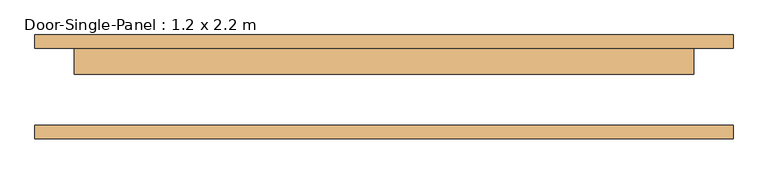
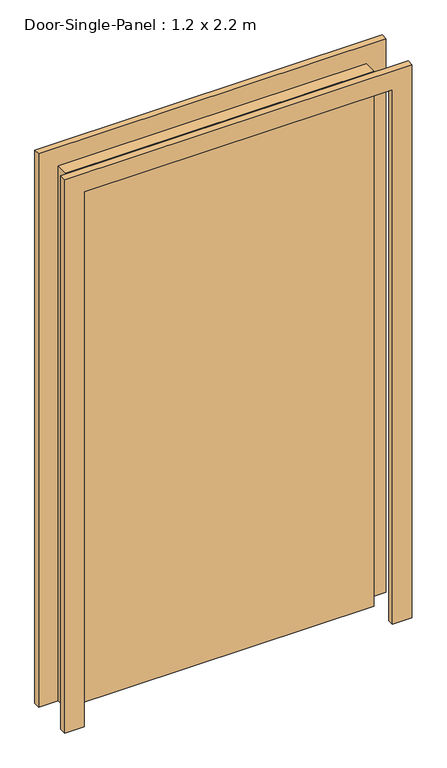
"""IFC4 building model written with IfcOpenShell, lengths in millimetres: door geometry, Door-Single-Panel : 1.2 x 2.2 m."""

import ifcopenshell
import ifcopenshell.guid

model = None  # the IFC model being written
_history = None  # IfcOwnerHistory: only IFC2X3 demands one
_inside = {}  # id of a spatial element -> (the spatial element, [elements in it])
_under = {}  # id of a project, library or spatial element -> (it, [spatial elements below it])
_declared = {}  # id of a project -> (the project, [libraries it declares])
_typed = {}  # id of a type object -> (the type object, [elements of that type])
_made_of = {}  # id of a material, layer set ... -> (it, [elements and type objects made of it])


def new_model(schema):
    """Start an empty IFC model of exactly this schema.

    Asked for "IFC4X3", IfcOpenShell would pick the latest addendum, in which some entities
    have other attributes; the version numbers below select the first issue.
    IFC2X3 requires an IfcOwnerHistory on every rooted entity: one is made here for all.
    """
    global model, _history
    if schema == "IFC4X3":
        model = ifcopenshell.file(schema_version=(4, 3, 0, 0))
    else:
        model = ifcopenshell.file(schema=schema)
    _inside.clear()
    _under.clear()
    _declared.clear()
    _typed.clear()
    _made_of.clear()
    _history = None
    if model.schema == "IFC2X3":
        org = make("IfcOrganization", Name="unknown")
        user = make(
            "IfcPersonAndOrganization",
            ThePerson=make("IfcPerson", FamilyName="unknown"),
            TheOrganization=org,
        )
        app = make(
            "IfcApplication",
            ApplicationDeveloper=org,
            Version="unknown",
            ApplicationFullName="unknown",
            ApplicationIdentifier="unknown",
        )
        _history = make(
            "IfcOwnerHistory",
            OwningUser=user,
            OwningApplication=app,
            ChangeAction="ADDED",
            CreationDate=0,
        )
    return model


def make(cls, **values):
    """One entity of the class cls with the attributes given. An attribute that is None is left unset."""
    return model.create_entity(
        cls, **{name: value for name, value in values.items() if value is not None}
    )


def rooted(cls, **values):
    """An entity with a GlobalId (a new one), such as an element, a storey or a relation."""
    return make(cls, GlobalId=ifcopenshell.guid.new(), OwnerHistory=_history, **values)


def si_unit(unit_type, name, prefix=None):
    """IfcSIUnit, for example si_unit("LENGTHUNIT", "METRE", prefix="MILLI")."""
    return make("IfcSIUnit", UnitType=unit_type, Prefix=prefix, Name=name)


def assignment(units):
    """IfcUnitAssignment: the units of a project."""
    return None if units is None else make("IfcUnitAssignment", Units=units)


def point(xyz):
    """IfcCartesianPoint."""
    return None if xyz is None else make("IfcCartesianPoint", Coordinates=xyz)


def direction(xyz):
    """IfcDirection."""
    return None if xyz is None else make("IfcDirection", DirectionRatios=xyz)


def frame(location, z_axis=None, x_axis=None):
    """IfcAxis2Placement3D, a coordinate frame: its origin and axes. An axis left out is left unset."""
    return make(
        "IfcAxis2Placement3D",
        Location=point(location),
        Axis=direction(z_axis),
        RefDirection=direction(x_axis),
    )


def origin():
    """The frame at (0, 0, 0) with its axes left unset."""
    return frame((0.0, 0.0, 0.0))


def origin_with_axes():
    """The frame at (0, 0, 0) with the z axis (0, 0, 1) and the x axis (1, 0, 0) written out."""
    return frame((0.0, 0.0, 0.0), z_axis=(0.0, 0.0, 1.0), x_axis=(1.0, 0.0, 0.0))


def place(relative_to, where):
    """IfcLocalPlacement: puts the frame where relative to a parent placement (None: the world)."""
    return make(
        "IfcLocalPlacement", PlacementRelTo=relative_to, RelativePlacement=where
    )


def context(
    kind, dimensions, precision=None, world=None, true_north=None, identifier=None
):
    """IfcGeometricRepresentationContext, for example the 3D "Model" context."""
    return make(
        "IfcGeometricRepresentationContext",
        ContextIdentifier=identifier,
        ContextType=kind,
        CoordinateSpaceDimension=dimensions,
        Precision=precision,
        WorldCoordinateSystem=world,
        TrueNorth=true_north,
    )


def project(units=None, contexts=None):
    """IfcProject with its units and contexts."""
    return rooted(
        "IfcProject",
        Name="project",
        RepresentationContexts=contexts,
        UnitsInContext=assignment(units),
    )


def spatial(cls, under=None, at=None, **own):
    """A site, building, storey or space (cls), placed at a placement, below another one or the project."""
    s = rooted(cls, ObjectPlacement=at, **own)
    if under is not None:
        _under.setdefault(under.id(), (under, []))[1].append(s)
    return s


def polyline(points):
    """IfcPolyline through the points."""
    return make("IfcPolyline", Points=[point(p) for p in points])


def outline(outer, holes=None, kind="AREA"):
    """IfcArbitraryClosedProfileDef: a profile drawn as a closed curve; with holes, ...WithVoids."""
    if holes is None:
        return make("IfcArbitraryClosedProfileDef", ProfileType=kind, OuterCurve=outer)
    return make(
        "IfcArbitraryProfileDefWithVoids",
        ProfileType=kind,
        OuterCurve=outer,
        InnerCurves=holes,
    )


def extrude(swept, where, along, depth):
    """IfcExtrudedAreaSolid: the profile swept, set in the frame where, extruded along a direction by depth."""
    return make(
        "IfcExtrudedAreaSolid",
        SweptArea=swept,
        Position=where,
        ExtrudedDirection=direction(along),
        Depth=depth,
    )


def shape(context_of_items, identifier, shape_type, items):
    """IfcShapeRepresentation: the items that make up one representation, for example the "Body"."""
    return make(
        "IfcShapeRepresentation",
        ContextOfItems=context_of_items,
        RepresentationIdentifier=identifier,
        RepresentationType=shape_type,
        Items=items,
    )


def source(mapping_origin, context_of_items, identifier, shape_type, items):
    """IfcRepresentationMap: a shape defined once, which mapped items show again and again."""
    return make(
        "IfcRepresentationMap",
        MappingOrigin=mapping_origin,
        MappedRepresentation=shape(context_of_items, identifier, shape_type, items),
    )


def transform(
    local_origin,
    x_axis=None,
    y_axis=None,
    z_axis=None,
    scale=None,
    scale2=None,
    scale3=None,
    uniform=True,
):
    """IfcCartesianTransformationOperator3D, or its non-uniform kind. x_axis, y_axis, z_axis: its Axis1, 2, 3."""
    if uniform:
        return make(
            "IfcCartesianTransformationOperator3D",
            Axis1=direction(x_axis),
            Axis2=direction(y_axis),
            LocalOrigin=point(local_origin),
            Scale=scale,
            Axis3=direction(z_axis),
        )
    return make(
        "IfcCartesianTransformationOperator3DnonUniform",
        Axis1=direction(x_axis),
        Axis2=direction(y_axis),
        LocalOrigin=point(local_origin),
        Scale=scale,
        Axis3=direction(z_axis),
        Scale2=scale2,
        Scale3=scale3,
    )


def mapped(mapping_source, mapping_target):
    """IfcMappedItem: shows the shape of a source again, moved by a transform."""
    return make(
        "IfcMappedItem", MappingSource=mapping_source, MappingTarget=mapping_target
    )


def made_of(thing, what):
    """Note that an element or type object is made of a material, layer set ...; save() writes the relation."""
    if what is not None:
        _made_of.setdefault(what.id(), (what, []))[1].append(thing)
    return thing


def element(
    cls,
    number,
    at=None,
    inside=None,
    cuts=None,
    type_object=None,
    material=None,
    context=None,
    identifier="Body",
    shape_type=None,
    held_by="IfcProductDefinitionShape",
    body=None,
    shapes=None,
    **own,
):
    """One element of the class cls, such as IfcWall. Its Tag is "e" and its number.

    at: its placement. inside: the storey or other place that contains it. cuts: it is an
    opening in that element (IfcRelVoidsElement). A single representation is given by context,
    identifier, shape_type and body (its items); several are given by shapes. held_by: the class
    of the entity that holds the representations. save() writes the other relations.
    """
    e = rooted(cls, Tag="e%d" % number, ObjectPlacement=at, **own)
    if body is not None:
        shapes = [shape(context, identifier, shape_type, body)]
    if shapes is not None:
        e.Representation = make(held_by, Representations=shapes)
    if inside is not None:
        _inside.setdefault(inside.id(), (inside, []))[1].append(e)
    if cuts is not None:
        rooted(
            "IfcRelVoidsElement", RelatingBuildingElement=cuts, RelatedOpeningElement=e
        )
    if type_object is not None:
        _typed.setdefault(type_object.id(), (type_object, []))[1].append(e)
    return made_of(e, material)


def aggregate(whole, parts):
    """IfcRelAggregates: a whole, such as a stair, and the parts it consists of."""
    return rooted("IfcRelAggregates", RelatingObject=whole, RelatedObjects=parts)


def save(model, path):
    """Write the relations noted so far, then the file.

    IfcRelAggregates (storeys below a building ...), IfcRelContainedInSpatialStructure (elements
    in a storey), IfcRelDefinesByType, IfcRelAssociatesMaterial and IfcRelDeclares: one each for
    every whole, place, type object, material and project.
    """
    for whole, parts in _under.values():
        aggregate(whole, parts)
    for where, things in _inside.values():
        rooted(
            "IfcRelContainedInSpatialStructure",
            RelatedElements=things,
            RelatingStructure=where,
        )
    for kind, things in _typed.values():
        rooted("IfcRelDefinesByType", RelatedObjects=things, RelatingType=kind)
    for what, things in _made_of.values():
        rooted("IfcRelAssociatesMaterial", RelatedObjects=things, RelatingMaterial=what)
    for by, libraries in _declared.values():
        rooted("IfcRelDeclares", RelatingContext=by, RelatedDefinitions=libraries)
    model.write(path)


def door_single_panel_1_2_x_2_2_m_37493633(model_context):
    return source(origin(), model_context, "Body", "SweptSolid", [
        extrude(outline(polyline([(600.0, 24.2), (-600.0, 24.2), (-600.0, 75.0), (600.0, 75.0), (600.0, 24.2)])), origin_with_axes(), (0.0, 0.0, 1.0), 2200.0),
        extrude(outline(polyline([(2276.2, 676.2), (2276.2, -676.2), (0.0, -676.2), (0.0, -600.0), (2200.0, -600.0), (2200.0, 600.0), (0.0, 600.0), (0.0, 676.2), (2276.2, 676.2)])), frame((0.0, -100.4, 0.0), z_axis=(0.0, 1.0, 0.0), x_axis=(0.0, 0.0, 1.0)), (0.0, 0.0, 1.0), 25.4),
        extrude(outline(polyline([(2276.2, -676.2), (0.0, -676.2), (0.0, -600.0), (2200.0, -600.0), (2200.0, 600.0), (0.0, 600.0), (0.0, 676.2), (2276.2, 676.2), (2276.2, -676.2)])), frame((0.0, 75.0, 0.0), z_axis=(0.0, 1.0, 0.0), x_axis=(0.0, 0.0, 1.0)), (0.0, 0.0, 1.0), 25.4),
    ])


if __name__ == "__main__":
    model = new_model("IFC4")
    model_context = context("Model", 3, world=origin())
    ifc_project = project(units=[si_unit("LENGTHUNIT", "METRE", prefix="MILLI")], contexts=[model_context])
    site = spatial("IfcSite", under=ifc_project)
    building = spatial("IfcBuilding", under=site)
    placement = place(None, origin())
    door_single_panel_1_2_x_2_2_m_shape = door_single_panel_1_2_x_2_2_m_37493633(model_context)
    element("IfcDoor", 1, ObjectType="Door-Single-Panel : 1.2 x 2.2 m", at=placement, inside=building, context=model_context, shape_type="MappedRepresentation", body=[
        mapped(door_single_panel_1_2_x_2_2_m_shape, transform((0.0, 0.0, 0.0), x_axis=(1.0, 0.0, 0.0), y_axis=(0.0, 1.0, 0.0), z_axis=(0.0, 0.0, 1.0))),
    ])
    save(model, "model.ifc")

# Revit data of these elements
# Type "Door-Single-Panel : 1.2 x 2.2 m"
#   Type Mark = "47"
#   Construction Type Id = "DOOR"
#   Analytic Construction = "Wooden"
#   Thickness = 0.0508 m
#   Thermal Resistance (R) = 0.455703 (m²·K)/W
#   Swing Angle [instance default] = 90.00°
#   Heat Transfer Coefficient (U) = 2.19465 W/(m²·K)
#   Height = 2.2 m
#   Trim Projection Ext = 0.0254 m
#   Trim Projection Int = 0.0254 m
#   Trim Width = 0.0762 m
#   Width = 1.2 m
#   Define Thermal Properties by = 1
#   Panel Material = Wood - Birch - Solid Stained Light Low Gloss
#   Trim Material = Paint - Sienna
#   Visual Light Transmittance = 0
#   Solar Heat Gain Coefficient = 0
#   Function = (empty or 0)
#   Wall Closure = (empty or 0)
# Element 1 (IfcDoor, "Door-Single-Panel : 1.2 x 2.2 m")
#   Materials on its faces: "Paint - Sienna", "Wood - Birch - Solid Stained Light Low Gloss"
# Materials
#   "Wood - Birch - Solid Stained Light Low Gloss": class "Wood", colour RGB 210 159 95, transparency 0, Cost = 0
#   "Paint - Sienna": class "Miscellaneous", colour RGB 118 70 51, transparency 0, Cost = 0
